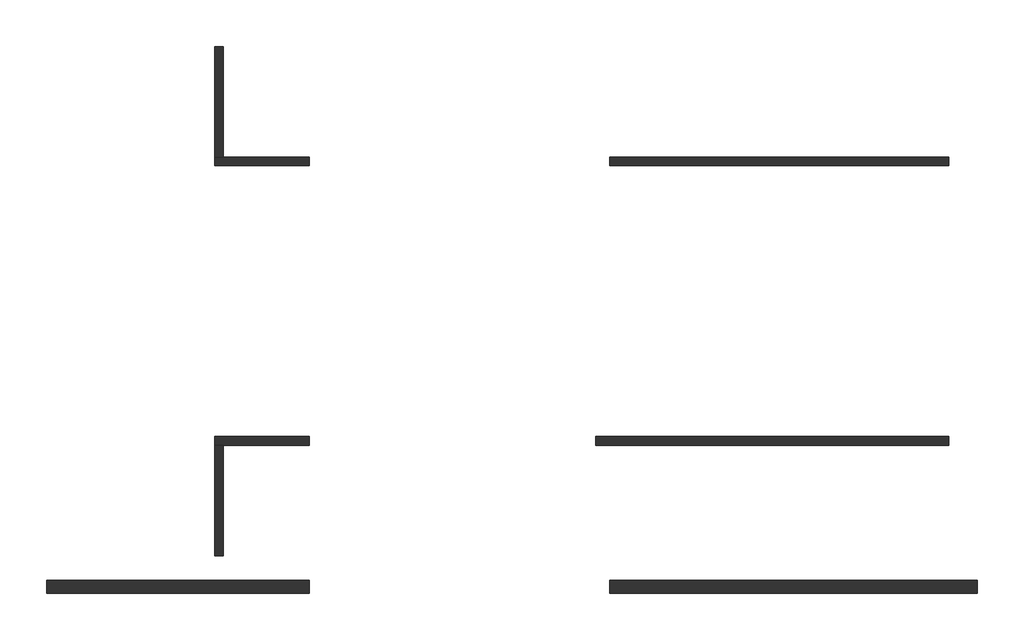
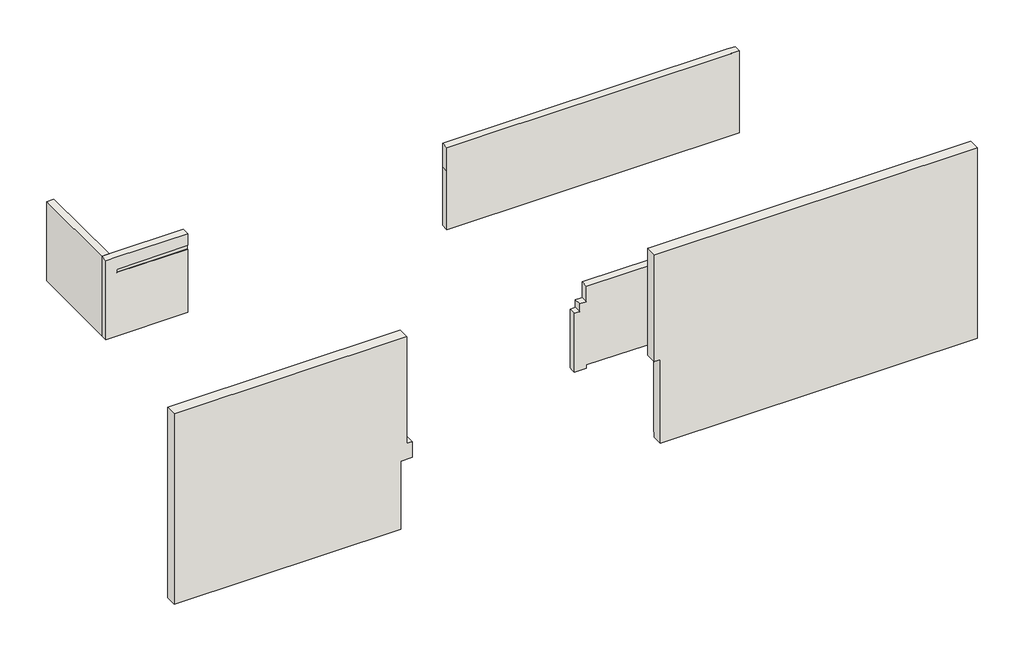
# One storey: 8 walls.
"""IFC4 building model written with IfcOpenShell, lengths in millimetres."""

from ifc_helpers import new_model, si_unit, frame, origin, place, context, project, spatial, polyline, outline, extrude, faceted_brep, element, save

model = new_model("IFC4")

# Units and contexts
model_context = context("Model", 3, world=origin())
ifc_project = project(units=[si_unit("LENGTHUNIT", "METRE", prefix="MILLI")], contexts=[model_context])

# Site, building, storey
site = spatial("IfcSite", under=ifc_project)
building = spatial("IfcBuilding", under=site)
storey = spatial("IfcBuildingStorey", under=building, Name="E-ACCESO", Elevation=-200.0)

# Walls
placement = place(None, origin())
element("IfcWall", 1, ObjectType="MURO TIPO 1_EXTERIOR_PETO_PABLO", at=placement, inside=storey, context=model_context, shape_type="Brep", body=[
    faceted_brep([(-11990.0, -17797.5, 7150.0), (-11975.0, -17797.5, 7150.0), (-205.0, -17797.5, 7150.0), (-205.0, -17797.5, -29.8903052), (-4292.2906333, -17797.5, 0.0), (-8394.5812666, -17797.5, -30.0), (-11770.0, -17797.5, 0.0), (-11770.0, -17797.5, 3030.0), (-11990.0, -17797.5, 3030.0), (-11770.0, -18207.5, -200.0), (-205.0, -18207.5, -200.0), (-205.0, -18207.5, 7150.0), (-11975.0, -18207.5, 7150.0), (-11990.0, -18207.5, 7150.0), (-11990.0, -18207.5, 3030.0), (-11975.0, -18207.5, 3030.0), (-11770.0, -18207.5, 3030.0), (-11770.0, -18207.5, 2430.0), (-11770.0, -17810.0, -200.0), (-205.0, -17810.0, -200.0), (-205.0, -17810.0, -29.8903052), (-8394.5812666, -17810.0, -30.0), (-4292.2906333, -17810.0, 0.0), (-11770.0, -17810.0, 0.0)], [[[0, 1, 2, 3, 4, 5, 6, 7, 8]], [[9, 10, 11, 12, 13, 14, 15, 16, 17]], [[10, 9, 18, 19]], [[2, 1, 0, 13, 12, 11]], [[2, 11, 10, 19, 20, 3]], [[21, 22, 20, 19, 18, 23]], [[20, 22, 4, 3]], [[21, 23, 6, 5]], [[22, 21, 5, 4]], [[13, 0, 8, 14]], [[14, 8, 7, 16, 15]], [[16, 7, 6, 23, 18, 9, 17]]]),
])
element("IfcWall", 2, ObjectType="MURO TIPO 5_PABLO", at=placement, inside=storey, context=model_context, shape_type="Brep", body=[
    faceted_brep([(-24205.0, -13267.5, 3030.0), (-23795.0, -13267.5, 3030.0), (-21230.0, -13267.5, 3030.0), (-20750.0, -13267.5, 3030.0), (-20750.0, -13267.5, 2430.0), (-20790.0, -13267.5, 2430.0), (-21215.0, -13267.5, 2430.0), (-21215.0, -13267.5, 2581.2), (-23795.0, -13267.5, 2551.3734104), (-23810.0, -13267.5, 2551.2), (-23810.0, -13267.5, 2430.0), (-23795.0, -13267.5, 2430.0), (-21230.0, -13267.5, 2430.0), (-21230.0, -13267.5, 0.0), (-24205.0, -13267.5, -28.0660377), (-24205.0, -13267.5, 2130.0), (-20750.0, -13537.5, 3030.0), (-20820.0, -13537.5, 3030.0), (-21230.0, -13537.5, 3030.0), (-23935.0, -13537.5, 3030.0), (-24205.0, -13537.5, 3030.0), (-24205.0, -13537.5, -28.0660377), (-23935.0, -13537.5, -25.5188679), (-21230.0, -13537.5, 0.0), (-21230.0, -13537.5, 2430.0), (-20820.0, -13537.5, 2430.0), (-20750.0, -13537.5, 2430.0), (-23810.0, -13282.5, 2430.0), (-21230.0, -13282.5, 2430.0), (-23810.0, -13282.5, 2551.2), (-21215.0, -13282.5, 2581.2), (-21215.0, -13282.5, 2430.0)], [[[0, 1, 2, 3, 4, 5, 6, 7, 8, 9, 10, 11, 12, 13, 14, 15]], [[16, 17, 18, 19, 20, 21, 22, 23, 24, 25, 26]], [[3, 2, 1, 0, 20, 19, 18, 17, 16]], [[20, 0, 15, 14, 21]], [[27, 28, 12, 11, 10]], [[29, 27, 10, 9]], [[27, 29, 30, 31, 28]], [[30, 29, 9, 8, 7]], [[14, 13, 23, 22, 21]], [[26, 25, 24, 28, 31, 6, 5, 4]], [[13, 12, 28, 24, 23]], [[4, 3, 16, 26]], [[31, 30, 7, 6]]]),
])
element("IfcWall", 3, ObjectType="MURO TIPO 5_PABLO", at=placement, inside=storey, context=model_context, shape_type="SweptSolid", body=[
    extrude(outline(polyline([(3030.0, -23935.0), (3030.0, -24205.0), (-28.0660377, -24205.0), (-25.5188679, -23935.0), (3030.0, -23935.0)])), frame((0.0, -17017.5, 0.0), z_axis=(0.0, 1.0, 0.0), x_axis=(0.0, 0.0, 1.0)), (0.0, 0.0, 1.0), 3480.0),
])
element("IfcWall", 4, ObjectType="MURO TIPO 5_PETO CUB_PABLO", at=placement, inside=storey, context=model_context, shape_type="Brep", body=[
    faceted_brep([(-1110.0, -13537.5, -23.2720515), (-1110.0, -13537.5, 3030.0), (-1380.0, -13537.5, 3030.0), (-1395.1532376, -13537.5, 3030.0), (-1410.1532376, -13537.5, 3030.0), (-1425.0, -13537.5, 3030.0), (-8795.0, -13537.5, 3030.0), (-9065.0, -13537.5, 3030.0), (-11770.0, -13537.5, 3030.0), (-11770.0, -13537.5, 2430.0), (-12010.0, -13537.5, 2430.0), (-12010.0, -13537.5, 2130.0), (-12210.0, -13537.5, 2130.0), (-12210.0, -13537.5, -135.0), (-11770.0, -13537.5, -135.0), (-11770.0, -13537.5, 0.0), (-9065.0, -13537.5, -24.0414616), (-8795.0, -13537.5, -26.4411639), (-8394.5812666, -13537.5, -30.0), (-4292.2906333, -13537.5, 0.0), (-1380.0, -13537.5, -21.2975449), (-1110.0, -13267.5, 3030.0), (-1110.0, -13267.5, -23.2720515), (-4292.2906333, -13267.5, 0.0), (-8394.5812666, -13267.5, -30.0), (-11770.0, -13267.5, 0.0), (-11770.0, -13267.5, -135.0), (-12210.0, -13267.5, -135.0), (-12210.0, -13267.5, 2100.0), (-12210.0, -13267.5, 2130.0), (-12010.0, -13267.5, 2130.0), (-12010.0, -13267.5, 2430.0), (-11785.0, -13267.5, 2430.0), (-11770.0, -13267.5, 2430.0), (-11770.0, -13267.5, 3030.0), (-9205.0, -13267.5, 3030.0), (-8795.0, -13267.5, 3030.0), (-1425.0, -13267.5, 3030.0), (-1410.1532376, -13267.5, 3030.0), (-1395.1532376, -13267.5, 3030.0), (-1380.0, -13267.5, 3030.0), (-12210.0, -13372.5, -135.0)], [[[0, 1, 2, 3, 4, 5, 6, 7, 8, 9, 10, 11, 12, 13, 14, 15, 16, 17, 18, 19, 20]], [[21, 22, 23, 24, 25, 26, 27, 28, 29, 30, 31, 32, 33, 34, 35, 36, 37, 38, 39, 40]], [[26, 14, 13, 41, 27]], [[1, 21, 40, 39, 38, 37, 36, 35, 34, 8, 7, 6, 5, 4, 3, 2]], [[21, 1, 0, 22]], [[0, 20, 19, 23, 22]], [[24, 18, 17, 16, 15, 25]], [[18, 24, 23, 19]], [[25, 15, 14, 26]], [[11, 30, 29, 12]], [[30, 11, 10, 31]], [[33, 32, 31, 10, 9]], [[27, 41, 13, 12, 29, 28]], [[8, 34, 33, 9]]]),
])
element("IfcWall", 5, ObjectType="MURO TIPO 5_PABLO", at=placement, inside=storey, context=model_context, shape_type="Brep", body=[
    faceted_brep([(-24205.0, -4462.5, 3030.0), (-23935.0, -4462.5, 3030.0), (-21230.0, -4462.5, 3030.0), (-21230.0, -4462.5, 0.0), (-23935.0, -4462.5, -25.5188679), (-24205.0, -4462.5, -28.0660377), (-21230.0, -4732.5, 3030.0), (-23795.0, -4732.5, 3030.0), (-24205.0, -4732.5, 3030.0), (-24205.0, -4732.5, 2130.0), (-24205.0, -4732.5, -28.0660377), (-21230.0, -4732.5, 0.0), (-21230.0, -4732.5, 2430.0), (-23795.0, -4732.5, 2430.0), (-23810.0, -4732.5, 2430.0), (-23810.0, -4732.5, 2551.2), (-23795.0, -4732.5, 2551.3734104), (-21230.0, -4732.5, 2581.0265896), (-21230.0, -4717.5, 2581.0265896), (-21230.0, -4717.5, 2430.0), (-23810.0, -4717.5, 2430.0), (-23810.0, -4717.5, 2551.2)], [[[0, 1, 2, 3, 4, 5]], [[6, 7, 8, 9, 10, 11, 12, 13, 14, 15, 16, 17]], [[2, 1, 0, 8, 7, 6]], [[2, 6, 17, 18, 19, 12, 11, 3]], [[8, 0, 5, 10, 9]], [[20, 14, 13, 12, 19]], [[21, 20, 19, 18]], [[20, 21, 15, 14]], [[21, 18, 17, 16, 15]], [[5, 4, 3, 11, 10]]]),
])
element("IfcWall", 6, ObjectType="MURO TIPO 5_PABLO", at=placement, inside=storey, context=model_context, shape_type="SweptSolid", body=[
    extrude(outline(polyline([(3030.0, -23935.0), (3030.0, -24205.0), (-28.0660377, -24205.0), (-25.5188679, -23935.0), (3030.0, -23935.0)])), frame((0.0, -4462.5, 0.0), z_axis=(0.0, 1.0, 0.0), x_axis=(0.0, 0.0, 1.0)), (0.0, 0.0, 1.0), 3480.0),
])
element("IfcWall", 7, ObjectType="MURO TIPO 5_PETO CUB_PABLO", at=placement, inside=storey, context=model_context, shape_type="Brep", body=[
    faceted_brep([(-11770.0, -4732.5, -135.0), (-1110.0, -4732.5, -135.0), (-1110.0, -4732.5, 3030.0), (-1380.0, -4732.5, 3030.0), (-1395.1532376, -4732.5, 3030.0), (-1410.1532376, -4732.5, 3030.0), (-1425.0, -4732.5, 3030.0), (-8795.0, -4732.5, 3030.0), (-9205.0, -4732.5, 3030.0), (-11770.0, -4732.5, 3030.0), (-11770.0, -4732.5, 2130.0), (-11770.0, -4732.5, 2100.0), (-11770.0, -4732.5, 0.0), (-1110.0, -4462.5, -135.0), (-11770.0, -4462.5, -135.0), (-11770.0, -4462.5, 2100.0), (-11770.0, -4462.5, 3030.0), (-9065.0, -4462.5, 3030.0), (-8795.0, -4462.5, 3030.0), (-1425.0, -4462.5, 3030.0), (-1410.1532376, -4462.5, 3030.0), (-1395.1532376, -4462.5, 3030.0), (-1380.0, -4462.5, 3030.0), (-1110.0, -4462.5, 3030.0), (-1110.0, -4462.5, -23.2720515)], [[[0, 1, 2, 3, 4, 5, 6, 7, 8, 9, 10, 11, 12]], [[13, 14, 15, 16, 17, 18, 19, 20, 21, 22, 23, 24]], [[1, 0, 14, 13]], [[2, 23, 22, 21, 20, 19, 18, 17, 16, 9, 8, 7, 6, 5, 4, 3]], [[2, 1, 13, 24, 23]], [[0, 12, 11, 15, 14]], [[9, 16, 15, 11, 10]]]),
])
element("IfcWall", 8, ObjectType="MURO TIPO 1_EXTERIOR_PETO_PABLO", at=placement, inside=storey, context=model_context, shape_type="Brep", body=[
    faceted_brep([(-21230.0, -17797.5, -200.0), (-29500.0, -17797.5, -200.0), (-29500.0, -17797.5, 0.0), (-29500.0, -17797.5, 7150.0), (-21025.0, -17797.5, 7150.0), (-21010.0, -17797.5, 7150.0), (-21010.0, -17797.5, 3030.0), (-20820.0, -17797.5, 3030.0), (-20820.0, -17797.5, 2430.0), (-21230.0, -17797.5, 2430.0), (-29500.0, -18207.5, -200.0), (-21230.0, -18207.5, -200.0), (-21230.0, -18207.5, 2430.0), (-20820.0, -18207.5, 2430.0), (-20820.0, -18207.5, 3030.0), (-21010.0, -18207.5, 3030.0), (-21010.0, -18207.5, 7150.0), (-21025.0, -18207.5, 7150.0), (-29500.0, -18207.5, 7150.0), (-29500.0, -18207.5, 0.0)], [[[0, 1, 2, 3, 4, 5, 6, 7, 8, 9]], [[10, 11, 12, 13, 14, 15, 16, 17, 18, 19]], [[1, 0, 11, 10]], [[3, 2, 1, 10, 19, 18]], [[5, 4, 3, 18, 17, 16]], [[5, 16, 15, 6]], [[0, 9, 12, 11]], [[8, 7, 14, 13]], [[13, 12, 9, 8]], [[6, 15, 14, 7]]]),
])

save(model, "model.ifc")

# Revit data of these elements
# Type "MURO TIPO 1_EXTERIOR_PETO_PABLO"
#   Keynote = "Md.1"
#   Description = "Muro interior-exterior perimetral"
#   Type Mark = "M1"
#   Layers, outside or top first: 0.015 m "Enfoscado cemento y pintura" (function 5); 0.115 m "Ladrillo cerámico perforado" (function 1); 0.15 m "Aire" (function 3); 0.115 m "Ladrillo cerámico perforado" (function 1); 0.015 m "Enfoscado cemento y pintura" (function 5)
# Type "MURO TIPO 5_PABLO"
#   Keynote = "Md.1"
#   Description = "Muro interior-interior patio exterior"
#   Type Mark = "M5"
#   Layers, outside or top first: 0.015 m "Enfoscado cemento y pintura" (function 5); 0.24 m "Ladrillo cerámico perforado" (function 1); 0.015 m "Enfoscado cemento y pintura" (function 5)
# Type "MURO TIPO 5_PETO CUB_PABLO"
#   Keynote = "Md.1"
#   Description = "Muro interior-interior patio exterior"
#   Type Mark = "M5"
#   Layers, outside or top first: 0.015 m "Enfoscado cemento y pintura" (function 5); 0.24 m "Ladrillo cerámico perforado" (function 1); 0.015 m "Enfoscado cemento y pintura" (function 5)
# Elements 1, 8 (IfcWall, "MURO TIPO 1_EXTERIOR_PETO_PABLO")
#   Top Offset = 0.00 m
#   Base Offset = 0.00 m
#   wall height = 7.35 m
#   Phase Created = Nueva construcción
#   Base Constraint = E-ACCESO
#   Top Constraint = AUXILIAR-CoronacionMuro
#   Materials on its faces: "Muro por defecto", "Enfoscado cemento y pintura"
# Element 2 (IfcWall, "MURO TIPO 5_PABLO")
#   built-in parameter 1001111 = 0.065 m
#   Top Offset = 0.00 m
#   Base Offset = 0.065 m
#   wall height = 3.165 m
#   Phase Created = Nueva construcción
#   Base Constraint = E-ACCESO
#   Top Constraint = AUXILIAR-Peto
#   Materials on its faces: "Muro por defecto", "Enfoscado cemento y pintura", "Enlucido de yeso"
# Elements 3, 5, 6 (IfcWall, "MURO TIPO 5_PABLO")
#   built-in parameter 1001111 = 0.065 m
#   Top Offset = 0.00 m
#   Base Offset = 0.065 m
#   wall height = 3.165 m
#   Phase Created = Nueva construcción
#   Base Constraint = E-ACCESO
#   Top Constraint = AUXILIAR-Peto
#   Materials on its faces: "Muro por defecto", "Enfoscado cemento y pintura"
# Element 4 (IfcWall, "MURO TIPO 5_PETO CUB_PABLO")
#   built-in parameter 1001111 = 0.065 m
#   Top Offset = 0.00 m
#   Base Offset = 0.065 m
#   wall height = 3.165 m
#   Phase Created = Nueva construcción
#   Base Constraint = E-ACCESO
#   Top Constraint = AUXILIAR-Peto
#   Materials on its faces: "Muro por defecto", "Enfoscado cemento y pintura", "Enlucido de yeso"
# Element 7 (IfcWall, "MURO TIPO 5_PETO CUB_PABLO")
#   built-in parameter 1001111 = 0.065 m
#   Top Offset = 0.00 m
#   Base Offset = 0.065 m
#   wall height = 3.165 m
#   Phase Created = Nueva construcción
#   Base Constraint = E-ACCESO
#   Top Constraint = AUXILIAR-Peto
#   Materials on its faces: "Muro por defecto", "Enfoscado cemento y pintura"
# Materials
#   "Enfoscado cemento y pintura": class "Varios", colour RGB 127 127 127, transparency 0, Keynote = "2", Comments = "Color blanco (1,5 cm)", Cost = 0
#   "Ladrillo cerámico perforado": class "Enladrillado", colour RGB 204 146 111, transparency 0, Cost = 0
#   "Aire": class "Gas", colour RGB 183 255 255, transparency 0.75, Description = "Aire", Cost = 0
#   "Muro por defecto": class "Varios", colour RGB 212 212 212, transparency 0, Cost = 0
#   "Enlucido de yeso": class "Placa de yeso laminado", colour RGB 249 249 249, transparency 0, Keynote = "1", Comments = "Color blanco al temple (1,5 cm)", Description = "1", Cost = 0
